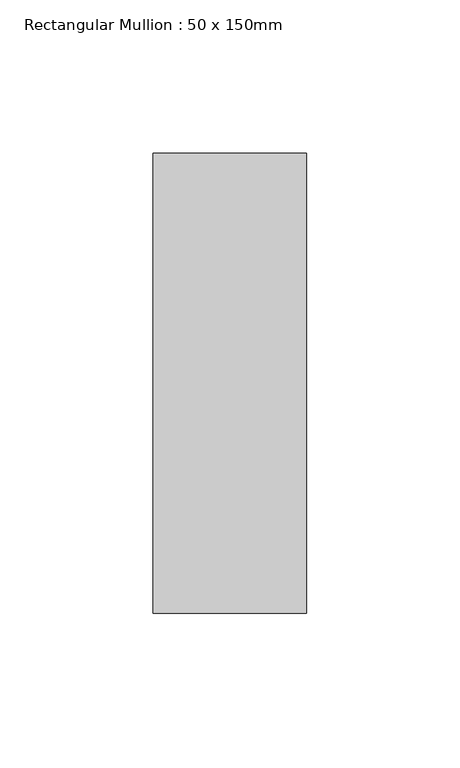
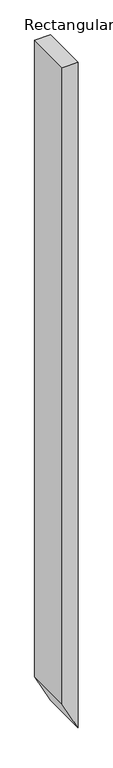
"""IFC4 building model written with IfcOpenShell, lengths in millimetres: member geometry, Rectangular Mullion : 50 x 150mm."""

from ifc_helpers import new_model, si_unit, frame, origin, place, context, project, spatial, polyline, outline, extrude, source, transform, mapped, element, save


def rectangular_mullion_50_x_150mm_2f01cdb9(model_context):
    return source(origin(), model_context, "Body", "SweptSolid", [
        extrude(outline(polyline([(0.0, 0.0), (0.0, -50.0), (-2114.4282315, -50.0), (-2210.4773379, 0.0), (0.0, 0.0)])), frame((0.0, -75.0, 0.0), z_axis=(0.0, 1.0, 0.0), x_axis=(0.0, 0.0, 1.0)), (0.0, 0.0, 1.0), 150.0),
    ])


if __name__ == "__main__":
    model = new_model("IFC4")
    model_context = context("Model", 3, world=origin())
    ifc_project = project(units=[si_unit("LENGTHUNIT", "METRE", prefix="MILLI")], contexts=[model_context])
    site = spatial("IfcSite", under=ifc_project)
    building = spatial("IfcBuilding", under=site)
    placement = place(None, origin())
    rectangular_mullion_50_x_150mm_shape = rectangular_mullion_50_x_150mm_2f01cdb9(model_context)
    element("IfcMember", 1, ObjectType="Rectangular Mullion : 50 x 150mm", at=placement, inside=building, context=model_context, shape_type="MappedRepresentation", body=[
        mapped(rectangular_mullion_50_x_150mm_shape, transform((0.0, 0.0, 0.0), x_axis=(1.0, 0.0, 0.0), y_axis=(0.0, 1.0, 0.0), z_axis=(0.0, 0.0, 1.0))),
    ])
    save(model, "model.ifc")

# Revit data of these elements
# Type "Rectangular Mullion : 50 x 150mm"
#   built-in parameter 1007304 = 0.492126 (stored number, unit not read)
#   built-in parameter 1007301 = 0.082021 (stored number, unit not read)
#   built-in parameter 1007300 = 0.082021 (stored number, unit not read)
# Element 1 (IfcMember, "Rectangular Mullion : 50 x 150mm")
#   Materials on its faces: "Aluminium"
# Materials
#   "Aluminium": class "Metal", colour RGB 247 247 247, transparency 0, Description = "Aluminium 6061", Cost = 0
